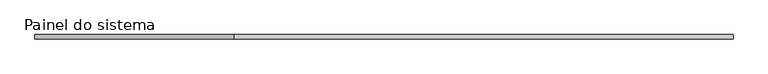
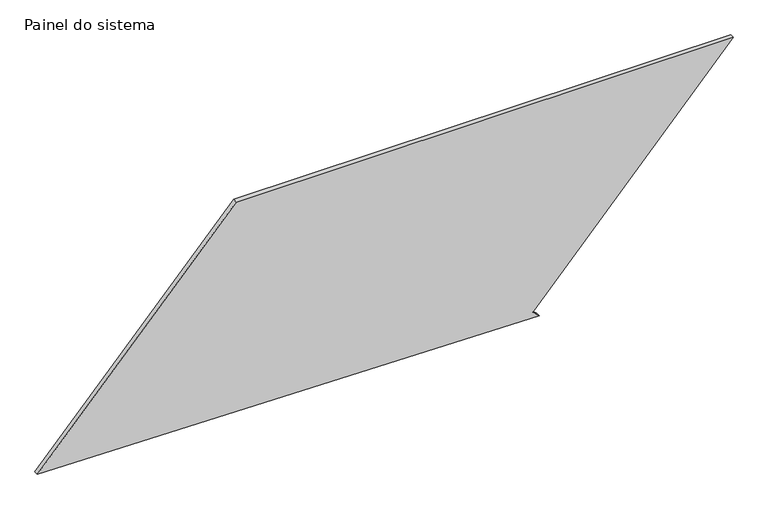
"""IFC4 building model written with IfcOpenShell, lengths in millimetres: plate geometry, Painel do sistema : Envidraçado."""

from ifc_helpers import new_model, si_unit, frame, origin, place, context, project, spatial, polyline, outline, extrude, source, transform, mapped, element, save


def painel_do_sistema_6644cb93(model_context):
    return source(origin(), model_context, "Body", "SweptSolid", [
        extrude(outline(polyline([(0.0, 863.5377747), (33.6679196, 826.5719637), (1269.1934048, 1951.8704906), (1269.1934048, -836.9974323), (45.1145996, -1951.8704906), (0.0, 863.5377747)])), frame((0.0, 24.5, 0.0), z_axis=(0.0, 1.0, 0.0), x_axis=(0.0, 0.0, 1.0)), (0.0, 0.0, 1.0), 25.0),
    ])


if __name__ == "__main__":
    model = new_model("IFC4")
    model_context = context("Model", 3, world=origin())
    ifc_project = project(units=[si_unit("LENGTHUNIT", "METRE", prefix="MILLI")], contexts=[model_context])
    site = spatial("IfcSite", under=ifc_project)
    building = spatial("IfcBuilding", under=site)
    placement = place(None, origin())
    painel_do_sistema_shape = painel_do_sistema_6644cb93(model_context)
    element("IfcPlate", 1, ObjectType="Painel do sistema : Envidraçado", at=placement, inside=building, context=model_context, shape_type="MappedRepresentation", body=[
        mapped(painel_do_sistema_shape, transform((0.0, 0.0, 0.0), x_axis=(1.0, 0.0, 0.0), y_axis=(0.0, 1.0, 0.0), z_axis=(0.0, 0.0, 1.0))),
    ])
    save(model, "model.ifc")

# Revit data of these elements
# Type "Painel do sistema : Envidraçado"
#   Construction Type Id = "GSP4R"
#   Analytic Construction = "Vidraça única Pilkington 1/8 pol"
#   Visual Light Transmittance = 0.9
#   Solar Heat Gain Coefficient = 0.86
#   Heat Transfer Coefficient (U) = 6.7069 W/(m²·K)
# Element 1 (IfcPlate, "Painel do sistema : Envidraçado")
#   Materials on its faces: "Vidro"
# Materials
#   "Vidro": class "Vidro", colour RGB 0 128 192, transparency 0.9, Description = "Vidro de sílica", Cost = 0
